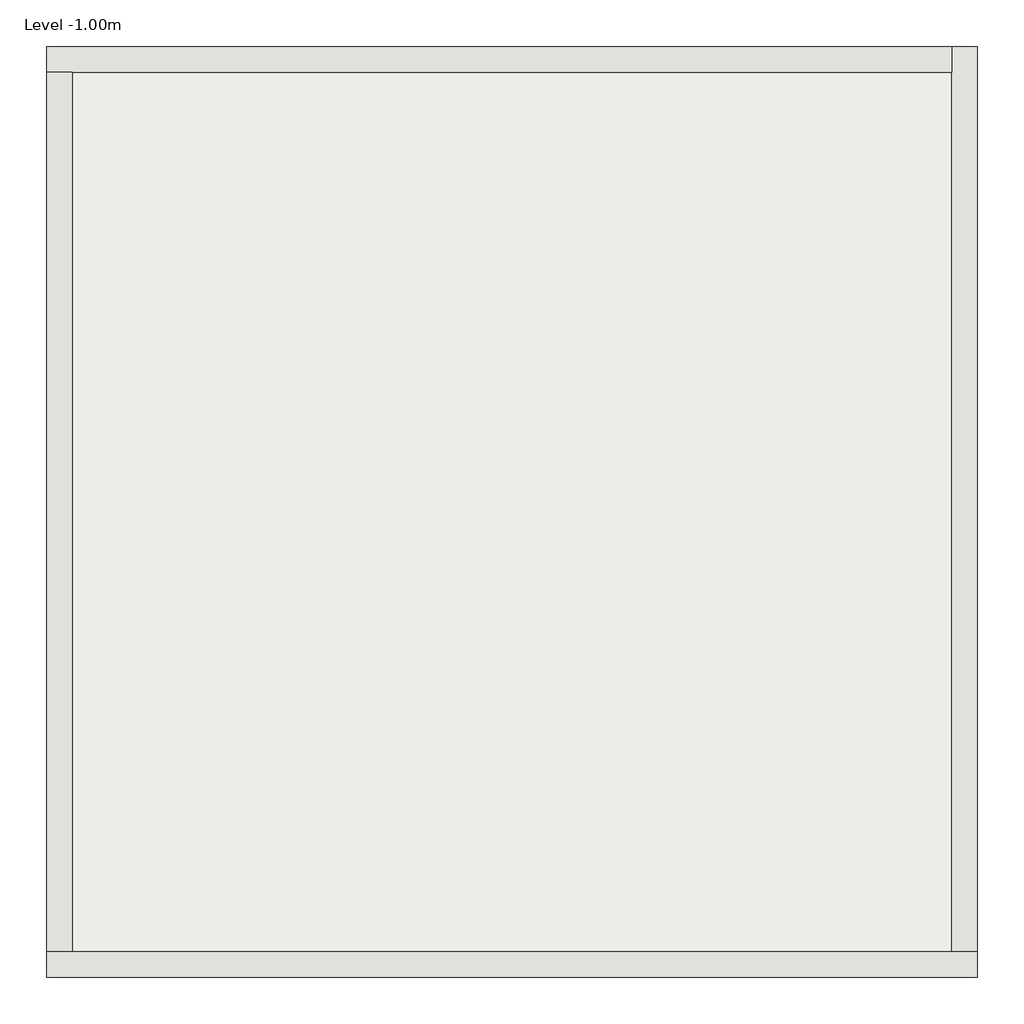
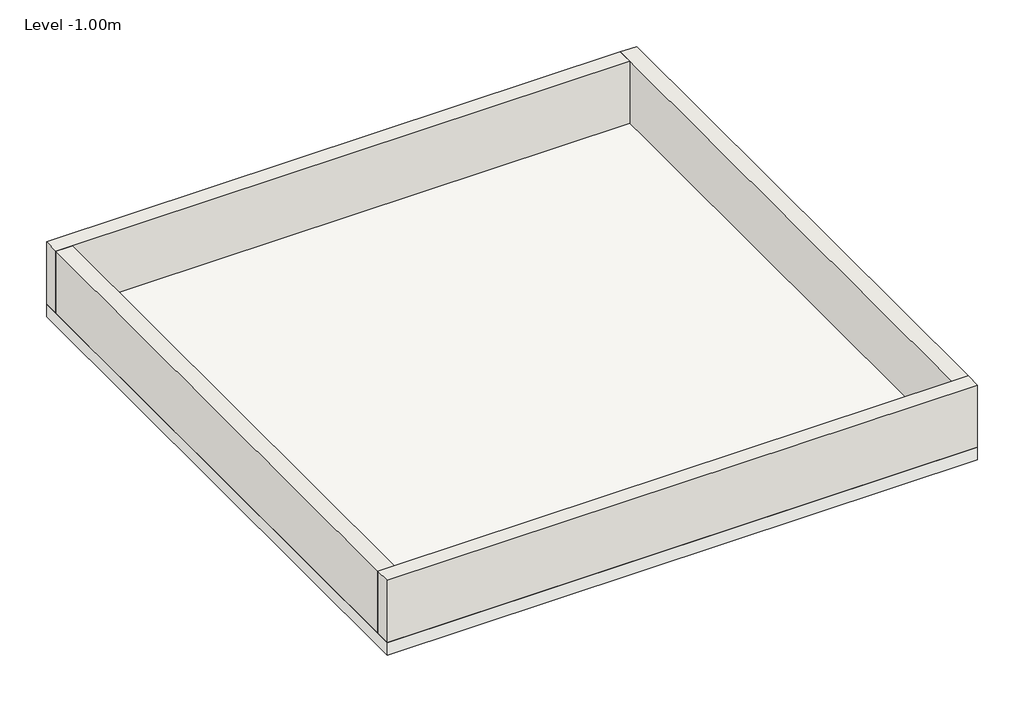
# One storey: 4 walls, 1 slab.
"""IFC4 building model written with IfcOpenShell, lengths in millimetres."""

import ifcopenshell
import ifcopenshell.guid

model = None  # the IFC model being written
_history = None  # IfcOwnerHistory: only IFC2X3 demands one
_inside = {}  # id of a spatial element -> (the spatial element, [elements in it])
_under = {}  # id of a project, library or spatial element -> (it, [spatial elements below it])
_declared = {}  # id of a project -> (the project, [libraries it declares])
_typed = {}  # id of a type object -> (the type object, [elements of that type])
_made_of = {}  # id of a material, layer set ... -> (it, [elements and type objects made of it])


def new_model(schema):
    """Start an empty IFC model of exactly this schema.

    Asked for "IFC4X3", IfcOpenShell would pick the latest addendum, in which some entities
    have other attributes; the version numbers below select the first issue.
    IFC2X3 requires an IfcOwnerHistory on every rooted entity: one is made here for all.
    """
    global model, _history
    if schema == "IFC4X3":
        model = ifcopenshell.file(schema_version=(4, 3, 0, 0))
    else:
        model = ifcopenshell.file(schema=schema)
    _inside.clear()
    _under.clear()
    _declared.clear()
    _typed.clear()
    _made_of.clear()
    _history = None
    if model.schema == "IFC2X3":
        org = make("IfcOrganization", Name="unknown")
        user = make(
            "IfcPersonAndOrganization",
            ThePerson=make("IfcPerson", FamilyName="unknown"),
            TheOrganization=org,
        )
        app = make(
            "IfcApplication",
            ApplicationDeveloper=org,
            Version="unknown",
            ApplicationFullName="unknown",
            ApplicationIdentifier="unknown",
        )
        _history = make(
            "IfcOwnerHistory",
            OwningUser=user,
            OwningApplication=app,
            ChangeAction="ADDED",
            CreationDate=0,
        )
    return model


def make(cls, **values):
    """One entity of the class cls with the attributes given. An attribute that is None is left unset."""
    return model.create_entity(
        cls, **{name: value for name, value in values.items() if value is not None}
    )


def rooted(cls, **values):
    """An entity with a GlobalId (a new one), such as an element, a storey or a relation."""
    return make(cls, GlobalId=ifcopenshell.guid.new(), OwnerHistory=_history, **values)


def si_unit(unit_type, name, prefix=None):
    """IfcSIUnit, for example si_unit("LENGTHUNIT", "METRE", prefix="MILLI")."""
    return make("IfcSIUnit", UnitType=unit_type, Prefix=prefix, Name=name)


def assignment(units):
    """IfcUnitAssignment: the units of a project."""
    return None if units is None else make("IfcUnitAssignment", Units=units)


def point(xyz):
    """IfcCartesianPoint."""
    return None if xyz is None else make("IfcCartesianPoint", Coordinates=xyz)


def direction(xyz):
    """IfcDirection."""
    return None if xyz is None else make("IfcDirection", DirectionRatios=xyz)


def frame(location, z_axis=None, x_axis=None):
    """IfcAxis2Placement3D, a coordinate frame: its origin and axes. An axis left out is left unset."""
    return make(
        "IfcAxis2Placement3D",
        Location=point(location),
        Axis=direction(z_axis),
        RefDirection=direction(x_axis),
    )


def origin():
    """The frame at (0, 0, 0) with its axes left unset."""
    return frame((0.0, 0.0, 0.0))


def place(relative_to, where):
    """IfcLocalPlacement: puts the frame where relative to a parent placement (None: the world)."""
    return make(
        "IfcLocalPlacement", PlacementRelTo=relative_to, RelativePlacement=where
    )


def context(
    kind, dimensions, precision=None, world=None, true_north=None, identifier=None
):
    """IfcGeometricRepresentationContext, for example the 3D "Model" context."""
    return make(
        "IfcGeometricRepresentationContext",
        ContextIdentifier=identifier,
        ContextType=kind,
        CoordinateSpaceDimension=dimensions,
        Precision=precision,
        WorldCoordinateSystem=world,
        TrueNorth=true_north,
    )


def project(units=None, contexts=None):
    """IfcProject with its units and contexts."""
    return rooted(
        "IfcProject",
        Name="project",
        RepresentationContexts=contexts,
        UnitsInContext=assignment(units),
    )


def spatial(cls, under=None, at=None, **own):
    """A site, building, storey or space (cls), placed at a placement, below another one or the project."""
    s = rooted(cls, ObjectPlacement=at, **own)
    if under is not None:
        _under.setdefault(under.id(), (under, []))[1].append(s)
    return s


def polyline(points):
    """IfcPolyline through the points."""
    return make("IfcPolyline", Points=[point(p) for p in points])


def outline(outer, holes=None, kind="AREA"):
    """IfcArbitraryClosedProfileDef: a profile drawn as a closed curve; with holes, ...WithVoids."""
    if holes is None:
        return make("IfcArbitraryClosedProfileDef", ProfileType=kind, OuterCurve=outer)
    return make(
        "IfcArbitraryProfileDefWithVoids",
        ProfileType=kind,
        OuterCurve=outer,
        InnerCurves=holes,
    )


def extrude(swept, where, along, depth):
    """IfcExtrudedAreaSolid: the profile swept, set in the frame where, extruded along a direction by depth."""
    return make(
        "IfcExtrudedAreaSolid",
        SweptArea=swept,
        Position=where,
        ExtrudedDirection=direction(along),
        Depth=depth,
    )


def faces_of(points, faces, orient=None, outer=None):
    """IfcFace entities. A face is a list of loops; a loop is a list of indices into points, from 0.

    orient and outer hold one flag for each loop. By default every Orientation is true, the
    first loop of a face is its IfcFaceOuterBound and the others are IfcFaceBound.
    """
    made = []
    for i, loops in enumerate(faces):
        bounds = []
        for j, loop in enumerate(loops):
            is_outer = j == 0 if outer is None else outer[i][j]
            bounds.append(
                make(
                    "IfcFaceOuterBound" if is_outer else "IfcFaceBound",
                    Bound=make("IfcPolyLoop", Polygon=[points[k] for k in loop]),
                    Orientation=True if orient is None else orient[i][j],
                )
            )
        made.append(make("IfcFace", Bounds=bounds))
    return made


def faceted_brep(points, faces, orient=None, outer=None, voids=None):
    """IfcFacetedBrep: a solid bounded by flat faces; with voids (closed shells), ...WithVoids."""
    shared = [point(p) for p in points]
    hull = make("IfcClosedShell", CfsFaces=faces_of(shared, faces, orient, outer))
    if voids is None:
        return make("IfcFacetedBrep", Outer=hull)
    return make(
        "IfcFacetedBrepWithVoids",
        Outer=hull,
        Voids=[
            make(cls, CfsFaces=faces_of(shared, fs, o, b)) for cls, fs, o, b in voids
        ],
    )


def shape(context_of_items, identifier, shape_type, items):
    """IfcShapeRepresentation: the items that make up one representation, for example the "Body"."""
    return make(
        "IfcShapeRepresentation",
        ContextOfItems=context_of_items,
        RepresentationIdentifier=identifier,
        RepresentationType=shape_type,
        Items=items,
    )


def made_of(thing, what):
    """Note that an element or type object is made of a material, layer set ...; save() writes the relation."""
    if what is not None:
        _made_of.setdefault(what.id(), (what, []))[1].append(thing)
    return thing


def element(
    cls,
    number,
    at=None,
    inside=None,
    cuts=None,
    type_object=None,
    material=None,
    context=None,
    identifier="Body",
    shape_type=None,
    held_by="IfcProductDefinitionShape",
    body=None,
    shapes=None,
    **own,
):
    """One element of the class cls, such as IfcWall. Its Tag is "e" and its number.

    at: its placement. inside: the storey or other place that contains it. cuts: it is an
    opening in that element (IfcRelVoidsElement). A single representation is given by context,
    identifier, shape_type and body (its items); several are given by shapes. held_by: the class
    of the entity that holds the representations. save() writes the other relations.
    """
    e = rooted(cls, Tag="e%d" % number, ObjectPlacement=at, **own)
    if body is not None:
        shapes = [shape(context, identifier, shape_type, body)]
    if shapes is not None:
        e.Representation = make(held_by, Representations=shapes)
    if inside is not None:
        _inside.setdefault(inside.id(), (inside, []))[1].append(e)
    if cuts is not None:
        rooted(
            "IfcRelVoidsElement", RelatingBuildingElement=cuts, RelatedOpeningElement=e
        )
    if type_object is not None:
        _typed.setdefault(type_object.id(), (type_object, []))[1].append(e)
    return made_of(e, material)


def aggregate(whole, parts):
    """IfcRelAggregates: a whole, such as a stair, and the parts it consists of."""
    return rooted("IfcRelAggregates", RelatingObject=whole, RelatedObjects=parts)


def save(model, path):
    """Write the relations noted so far, then the file.

    IfcRelAggregates (storeys below a building ...), IfcRelContainedInSpatialStructure (elements
    in a storey), IfcRelDefinesByType, IfcRelAssociatesMaterial and IfcRelDeclares: one each for
    every whole, place, type object, material and project.
    """
    for whole, parts in _under.values():
        aggregate(whole, parts)
    for where, things in _inside.values():
        rooted(
            "IfcRelContainedInSpatialStructure",
            RelatedElements=things,
            RelatingStructure=where,
        )
    for kind, things in _typed.values():
        rooted("IfcRelDefinesByType", RelatedObjects=things, RelatingType=kind)
    for what, things in _made_of.values():
        rooted("IfcRelAssociatesMaterial", RelatedObjects=things, RelatingMaterial=what)
    for by, libraries in _declared.values():
        rooted("IfcRelDeclares", RelatingContext=by, RelatedDefinitions=libraries)
    model.write(path)


model = new_model("IFC4")

# Units and contexts
model_context = context("Model", 3, world=origin())
ifc_project = project(units=[si_unit("LENGTHUNIT", "METRE", prefix="MILLI")], contexts=[model_context])

# Site, building, storey
site = spatial("IfcSite", under=ifc_project)
building = spatial("IfcBuilding", under=site)
storey = spatial("IfcBuildingStorey", under=building, Name="Level -1.00m", Elevation=-1000.0)

# Slab
placement = place(None, origin())
element("IfcSlab", 1, ObjectType="SOL CAM SANIT", at=placement, inside=storey, context=model_context, shape_type="SweptSolid", body=[
    extrude(outline(polyline([(0.0, 7999.9941531), (9000.0000251, 7999.9941531), (9000.0000251, -1000.0058651), (0.0, -1000.0058651), (0.0, 7999.9941531)])), frame((0.0, 0.0, -1202.9999956), z_axis=(0.0, 0.0, 1.0), x_axis=(1.0, 0.0, 0.0)), (0.0, 0.0, 1.0), 202.9999956),
])

# Walls
element("IfcWall", 2, ObjectType="MURO CAM SANIT", at=placement, inside=storey, context=model_context, shape_type="Brep", body=[
    faceted_brep([(6.9e-06, -1000.0058651, -1000.0), (9000.0000251, -1000.0058651, -1000.0), (9000.0000251, -1000.0058651, -0.01216), (6.9e-06, -1000.0058651, -0.01216), (6.9e-06, -751.0058709, -1000.0), (6.9e-06, -751.0058709, -0.01216), (249.0000011, -751.0058709, -0.01216), (8751.0000309, -751.0058709, -0.01216), (9000.0000251, -751.0058709, -0.01216), (9000.0000251, -751.0058709, -1000.0), (8751.0000309, -751.0058709, -1000.0), (249.0000011, -751.0058709, -1000.0)], [[[0, 1, 2, 3]], [[4, 5, 6, 7, 8, 9, 10, 11]], [[1, 0, 4, 11, 10, 9]], [[3, 2, 8, 7, 6, 5]], [[2, 1, 9, 8]], [[0, 3, 5, 4]]]),
])
element("IfcWall", 3, ObjectType="MURO CAM SANIT", at=placement, inside=storey, context=model_context, shape_type="Brep", body=[
    faceted_brep([(9000.0000251, -751.0058709, -1000.0), (9000.0000251, 7999.9941531, -1000.0), (9000.0000251, 7999.9941531, -0.01216), (9000.0000251, -751.0058709, -0.01216), (8751.0000309, -751.0058709, -1000.0), (8751.0000309, -751.0058709, -0.01216), (8751.0000309, 7750.9941589, -0.01216), (8751.0000309, 7999.9941531, -0.01216), (8751.0000309, 7999.9941531, -1000.0), (8751.0000309, 7750.9941589, -1000.0)], [[[0, 1, 2, 3]], [[4, 5, 6, 7, 8, 9]], [[1, 0, 4, 9, 8]], [[3, 2, 7, 6, 5]], [[2, 1, 8, 7]], [[0, 3, 5, 4]]]),
])
element("IfcWall", 4, ObjectType="MURO CAM SANIT", at=placement, inside=storey, context=model_context, shape_type="Brep", body=[
    faceted_brep([(8751.0000309, 7999.9941531, -1000.0), (6.9e-06, 7999.9941531, -1000.0), (6.9e-06, 7999.9941531, -0.01216), (8751.0000309, 7999.9941531, -0.01216), (8751.0000309, 7750.9941589, -1000.0), (8751.0000309, 7750.9941589, -0.01216), (249.0000011, 7750.9941589, -0.01216), (6.9e-06, 7750.9941589, -0.01216), (6.9e-06, 7750.9941589, -1000.0), (249.0000011, 7750.9941589, -1000.0)], [[[0, 1, 2, 3]], [[4, 5, 6, 7, 8, 9]], [[1, 0, 4, 9, 8]], [[3, 2, 7, 6, 5]], [[2, 1, 8, 7]], [[0, 3, 5, 4]]]),
])
element("IfcWall", 5, ObjectType="MURO CAM SANIT", at=placement, inside=storey, context=model_context, shape_type="SweptSolid", body=[
    extrude(outline(polyline([(6.9e-06, -751.0058709), (6.9e-06, 7750.9941589), (249.0000011, 7750.9941589), (249.0000011, -751.0058709), (6.9e-06, -751.0058709)])), frame((0.0, 0.0, -1000.0), z_axis=(0.0, 0.0, 1.0), x_axis=(1.0, 0.0, 0.0)), (0.0, 0.0, 1.0), 999.98784),
])

save(model, "model.ifc")

# Revit data of these elements
# Project information
#   Organization Name = "Organization Name"
#   Organization Description = "Organization Description"
#   Building Name = "Building Name"
#   Project Issue Date = "Issue Date"
#   Project Status = "Project Status"
#   Client Name = "Client Name"
#   Project Address = "Enter address here\nAddress Line 2"
#   Project Name = "Project Name"
#   Project Number = "Project Number"
# Type "SOL CAM SANIT"
#   Type Comments = "CTE"
#   Type Mark = "FS-01"
#   Layers, outside or top first: 0.080 m "Hormigón en masa d entre 2000 y 2300" (function 4); 0.003 m "Cloruro de polivinilo (PVC)" (function 4); 0.120 m "Arena y grava (d entre 1700 y 2200)" (function 1)
# Type "MURO CAM SANIT"
#   Type Comments = "CTE"
#   Description = "Metal Studs with Brick over sheathing on exterior and Gypsum Wall Board (GWB) on interior, Exterior Function"
#   Assembly Code = "B2010158"
#   Type Mark = "W-01"
#   Layers, outside or top first: 0.009 m "Betún fieltro o lámina" (function 4); 0.240 m "1 pie LP métrico o catalán 40 mm menor G menor 60 mm" (function 1)
# Element 1 (IfcSlab, "SOL CAM SANIT")
#   Height Offset From Level = 0.000 m
#   Phase Created = New Construction
#   Materials on its faces: "Arena y grava (d entre 1700 y 2200)", "Hormigón en masa d entre 2000 y 2300"
# Element 2 (IfcWall, "MURO CAM SANIT")
#   Comments = "BEM_GROUND_COUPLED"
#   Top Offset = 0.000 m
#   Base Offset = 0.000 m
#   Unconnected Height = 0.999988 m
#   wall height = 0.999988 m
#   Phase Created = New Construction
#   Base Constraint = Level -1.00m
#   Materials on its faces: "1 pie LP métrico o catalán 40 mm menor G menor 60 mm", "Default Wall", "Betún fieltro o lámina"
# Elements 3, 4, 5 (IfcWall, "MURO CAM SANIT")
#   Comments = "BEM_GROUND_COUPLED"
#   Top Offset = 0.000 m
#   Base Offset = 0.000 m
#   Unconnected Height = 0.999988 m
#   wall height = 0.999988 m
#   Phase Created = New Construction
#   Base Constraint = Level -1.00m
#   Materials on its faces: "Default Wall", "1 pie LP métrico o catalán 40 mm menor G menor 60 mm", "Betún fieltro o lámina"
# Materials
#   "Hormigón en masa d entre 2000 y 2300": class "Unassigned", colour RGB 0 0 0, transparency 0
#   "Cloruro de polivinilo (PVC)": class "Unassigned", colour RGB 0 0 0, transparency 0, Model = "0.170000001788", Comments = "Cp: 900 J/kgK", Description = "HULC Import | Density: 1390 kg/m3"
#   "Arena y grava (d entre 1700 y 2200)": class "Unassigned", colour RGB 0 0 0, transparency 0, Model = "2", Comments = "Cp: 1050 J/kgK", Description = "HULC Import | Density: 1450 kg/m3"
#   "Betún fieltro o lámina": class "Unassigned", colour RGB 0 0 0, transparency 0, Model = "0.23", Comments = "CTE"
#   "1 pie LP métrico o catalán 40 mm menor G menor 60 mm": class "Unassigned", colour RGB 0 0 0, transparency 0
#   "Default Wall": class "Miscellaneous", colour RGB 192 192 192, transparency 0, Cost = 0
# Space at (4084.009, 3345.189) mm, phase "New Construction", upper level "Level -1.00m", upper offset 1.000 m, lower offset 0.000 m
#   Number = "4"
#   Name = "Space"
#   Actual Lighting Load per area = 0
#   Actual Power Load per area = 0
#   Sensible Heat Gain per person = 0
#   Specified Lighting Load = 8374.95 (stored number, unit not read)
#   Specified Power Load = 10887.4 (stored number, unit not read)
#   Latent Heat Gain per person = 0
#   Total Heat Gain per person = 0
#   Area per Person = 0
#   Number of People = 2.52994 (stored number, unit not read)
#   Lighting Load Units = 0
#   Power Load Units = 0
#   Return Airflow = 0
#   Occupancy Unit = -1
#   Condition Type = 2
#   Construction Type = none
